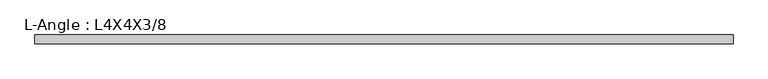
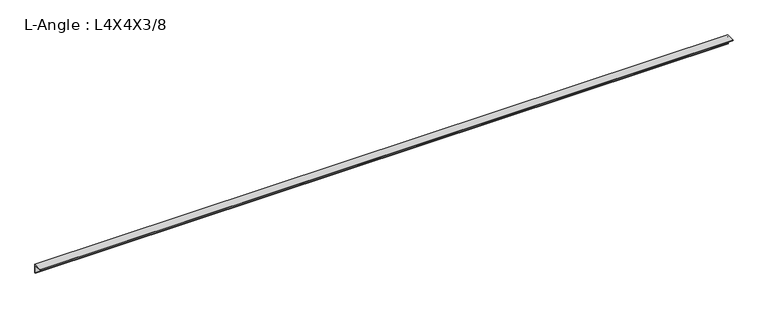
"""IFC4 building model written with IfcOpenShell, lengths in millimetres: beam geometry, L-Angle : L4X4X3/8."""

import ifcopenshell
import ifcopenshell.guid

model = None  # the IFC model being written
_history = None  # IfcOwnerHistory: only IFC2X3 demands one
_inside = {}  # id of a spatial element -> (the spatial element, [elements in it])
_under = {}  # id of a project, library or spatial element -> (it, [spatial elements below it])
_declared = {}  # id of a project -> (the project, [libraries it declares])
_typed = {}  # id of a type object -> (the type object, [elements of that type])
_made_of = {}  # id of a material, layer set ... -> (it, [elements and type objects made of it])


def new_model(schema):
    """Start an empty IFC model of exactly this schema.

    Asked for "IFC4X3", IfcOpenShell would pick the latest addendum, in which some entities
    have other attributes; the version numbers below select the first issue.
    IFC2X3 requires an IfcOwnerHistory on every rooted entity: one is made here for all.
    """
    global model, _history
    if schema == "IFC4X3":
        model = ifcopenshell.file(schema_version=(4, 3, 0, 0))
    else:
        model = ifcopenshell.file(schema=schema)
    _inside.clear()
    _under.clear()
    _declared.clear()
    _typed.clear()
    _made_of.clear()
    _history = None
    if model.schema == "IFC2X3":
        org = make("IfcOrganization", Name="unknown")
        user = make(
            "IfcPersonAndOrganization",
            ThePerson=make("IfcPerson", FamilyName="unknown"),
            TheOrganization=org,
        )
        app = make(
            "IfcApplication",
            ApplicationDeveloper=org,
            Version="unknown",
            ApplicationFullName="unknown",
            ApplicationIdentifier="unknown",
        )
        _history = make(
            "IfcOwnerHistory",
            OwningUser=user,
            OwningApplication=app,
            ChangeAction="ADDED",
            CreationDate=0,
        )
    return model


def make(cls, **values):
    """One entity of the class cls with the attributes given. An attribute that is None is left unset."""
    return model.create_entity(
        cls, **{name: value for name, value in values.items() if value is not None}
    )


def rooted(cls, **values):
    """An entity with a GlobalId (a new one), such as an element, a storey or a relation."""
    return make(cls, GlobalId=ifcopenshell.guid.new(), OwnerHistory=_history, **values)


def si_unit(unit_type, name, prefix=None):
    """IfcSIUnit, for example si_unit("LENGTHUNIT", "METRE", prefix="MILLI")."""
    return make("IfcSIUnit", UnitType=unit_type, Prefix=prefix, Name=name)


def assignment(units):
    """IfcUnitAssignment: the units of a project."""
    return None if units is None else make("IfcUnitAssignment", Units=units)


def point(xyz):
    """IfcCartesianPoint."""
    return None if xyz is None else make("IfcCartesianPoint", Coordinates=xyz)


def direction(xyz):
    """IfcDirection."""
    return None if xyz is None else make("IfcDirection", DirectionRatios=xyz)


def frame(location, z_axis=None, x_axis=None):
    """IfcAxis2Placement3D, a coordinate frame: its origin and axes. An axis left out is left unset."""
    return make(
        "IfcAxis2Placement3D",
        Location=point(location),
        Axis=direction(z_axis),
        RefDirection=direction(x_axis),
    )


def frame_2d(location, x_axis=None):
    """IfcAxis2Placement2D, a coordinate frame in the plane: its origin and x axis."""
    return make(
        "IfcAxis2Placement2D", Location=point(location), RefDirection=direction(x_axis)
    )


def origin():
    """The frame at (0, 0, 0) with its axes left unset."""
    return frame((0.0, 0.0, 0.0))


def place(relative_to, where):
    """IfcLocalPlacement: puts the frame where relative to a parent placement (None: the world)."""
    return make(
        "IfcLocalPlacement", PlacementRelTo=relative_to, RelativePlacement=where
    )


def context(
    kind, dimensions, precision=None, world=None, true_north=None, identifier=None
):
    """IfcGeometricRepresentationContext, for example the 3D "Model" context."""
    return make(
        "IfcGeometricRepresentationContext",
        ContextIdentifier=identifier,
        ContextType=kind,
        CoordinateSpaceDimension=dimensions,
        Precision=precision,
        WorldCoordinateSystem=world,
        TrueNorth=true_north,
    )


def project(units=None, contexts=None):
    """IfcProject with its units and contexts."""
    return rooted(
        "IfcProject",
        Name="project",
        RepresentationContexts=contexts,
        UnitsInContext=assignment(units),
    )


def spatial(cls, under=None, at=None, **own):
    """A site, building, storey or space (cls), placed at a placement, below another one or the project."""
    s = rooted(cls, ObjectPlacement=at, **own)
    if under is not None:
        _under.setdefault(under.id(), (under, []))[1].append(s)
    return s


def polyline(points):
    """IfcPolyline through the points."""
    return make("IfcPolyline", Points=[point(p) for p in points])


def circle_curve(where, radius):
    """IfcCircle in the frame where."""
    return make("IfcCircle", Position=where, Radius=radius)


def trimmed(basis, trim1, trim2, sense, master):
    """IfcTrimmedCurve: the piece of a basis curve between two trims."""
    return make(
        "IfcTrimmedCurve",
        BasisCurve=basis,
        Trim1=trim1,
        Trim2=trim2,
        SenseAgreement=sense,
        MasterRepresentation=master,
    )


def segment(curve, same_sense, transition):
    """IfcCompositeCurveSegment."""
    return make(
        "IfcCompositeCurveSegment",
        Transition=transition,
        SameSense=same_sense,
        ParentCurve=curve,
    )


def composite_curve(segments, self_intersect=None):
    """IfcCompositeCurve: segments joined end to end."""
    return make("IfcCompositeCurve", Segments=segments, SelfIntersect=self_intersect)


def outline(outer, holes=None, kind="AREA"):
    """IfcArbitraryClosedProfileDef: a profile drawn as a closed curve; with holes, ...WithVoids."""
    if holes is None:
        return make("IfcArbitraryClosedProfileDef", ProfileType=kind, OuterCurve=outer)
    return make(
        "IfcArbitraryProfileDefWithVoids",
        ProfileType=kind,
        OuterCurve=outer,
        InnerCurves=holes,
    )


def extrude(swept, where, along, depth):
    """IfcExtrudedAreaSolid: the profile swept, set in the frame where, extruded along a direction by depth."""
    return make(
        "IfcExtrudedAreaSolid",
        SweptArea=swept,
        Position=where,
        ExtrudedDirection=direction(along),
        Depth=depth,
    )


def shape(context_of_items, identifier, shape_type, items):
    """IfcShapeRepresentation: the items that make up one representation, for example the "Body"."""
    return make(
        "IfcShapeRepresentation",
        ContextOfItems=context_of_items,
        RepresentationIdentifier=identifier,
        RepresentationType=shape_type,
        Items=items,
    )


def source(mapping_origin, context_of_items, identifier, shape_type, items):
    """IfcRepresentationMap: a shape defined once, which mapped items show again and again."""
    return make(
        "IfcRepresentationMap",
        MappingOrigin=mapping_origin,
        MappedRepresentation=shape(context_of_items, identifier, shape_type, items),
    )


def transform(
    local_origin,
    x_axis=None,
    y_axis=None,
    z_axis=None,
    scale=None,
    scale2=None,
    scale3=None,
    uniform=True,
):
    """IfcCartesianTransformationOperator3D, or its non-uniform kind. x_axis, y_axis, z_axis: its Axis1, 2, 3."""
    if uniform:
        return make(
            "IfcCartesianTransformationOperator3D",
            Axis1=direction(x_axis),
            Axis2=direction(y_axis),
            LocalOrigin=point(local_origin),
            Scale=scale,
            Axis3=direction(z_axis),
        )
    return make(
        "IfcCartesianTransformationOperator3DnonUniform",
        Axis1=direction(x_axis),
        Axis2=direction(y_axis),
        LocalOrigin=point(local_origin),
        Scale=scale,
        Axis3=direction(z_axis),
        Scale2=scale2,
        Scale3=scale3,
    )


def mapped(mapping_source, mapping_target):
    """IfcMappedItem: shows the shape of a source again, moved by a transform."""
    return make(
        "IfcMappedItem", MappingSource=mapping_source, MappingTarget=mapping_target
    )


def made_of(thing, what):
    """Note that an element or type object is made of a material, layer set ...; save() writes the relation."""
    if what is not None:
        _made_of.setdefault(what.id(), (what, []))[1].append(thing)
    return thing


def element(
    cls,
    number,
    at=None,
    inside=None,
    cuts=None,
    type_object=None,
    material=None,
    context=None,
    identifier="Body",
    shape_type=None,
    held_by="IfcProductDefinitionShape",
    body=None,
    shapes=None,
    **own,
):
    """One element of the class cls, such as IfcWall. Its Tag is "e" and its number.

    at: its placement. inside: the storey or other place that contains it. cuts: it is an
    opening in that element (IfcRelVoidsElement). A single representation is given by context,
    identifier, shape_type and body (its items); several are given by shapes. held_by: the class
    of the entity that holds the representations. save() writes the other relations.
    """
    e = rooted(cls, Tag="e%d" % number, ObjectPlacement=at, **own)
    if body is not None:
        shapes = [shape(context, identifier, shape_type, body)]
    if shapes is not None:
        e.Representation = make(held_by, Representations=shapes)
    if inside is not None:
        _inside.setdefault(inside.id(), (inside, []))[1].append(e)
    if cuts is not None:
        rooted(
            "IfcRelVoidsElement", RelatingBuildingElement=cuts, RelatedOpeningElement=e
        )
    if type_object is not None:
        _typed.setdefault(type_object.id(), (type_object, []))[1].append(e)
    return made_of(e, material)


def aggregate(whole, parts):
    """IfcRelAggregates: a whole, such as a stair, and the parts it consists of."""
    return rooted("IfcRelAggregates", RelatingObject=whole, RelatedObjects=parts)


def save(model, path):
    """Write the relations noted so far, then the file.

    IfcRelAggregates (storeys below a building ...), IfcRelContainedInSpatialStructure (elements
    in a storey), IfcRelDefinesByType, IfcRelAssociatesMaterial and IfcRelDeclares: one each for
    every whole, place, type object, material and project.
    """
    for whole, parts in _under.values():
        aggregate(whole, parts)
    for where, things in _inside.values():
        rooted(
            "IfcRelContainedInSpatialStructure",
            RelatedElements=things,
            RelatingStructure=where,
        )
    for kind, things in _typed.values():
        rooted("IfcRelDefinesByType", RelatedObjects=things, RelatingType=kind)
    for what, things in _made_of.values():
        rooted("IfcRelAssociatesMaterial", RelatedObjects=things, RelatingMaterial=what)
    for by, libraries in _declared.values():
        rooted("IfcRelDeclares", RelatingContext=by, RelatedDefinitions=libraries)
    model.write(path)


def l_angle_l4x4x3_8_194fa828(model_context):
    return source(origin(), model_context, "Body", "SweptSolid", [
        extrude(outline(composite_curve([segment(polyline([(28.702, 28.702), (28.702, -72.898)]), True, "CONTINUOUS"), segment(trimmed(circle_curve(frame_2d((28.702, -63.373)), 9.525), [point((28.702, -72.898))], [point((19.177, -63.373))], False, "CARTESIAN"), True, "CONTINUOUS"), segment(polyline([(19.177, -63.373), (19.177, 9.652)]), True, "CONTINUOUS"), segment(trimmed(circle_curve(frame_2d((9.652, 9.652)), 9.525), [point((19.177, 9.652))], [point((9.652, 19.177))], True, "CARTESIAN"), True, "CONTINUOUS"), segment(polyline([(9.652, 19.177), (-63.373, 19.177)]), True, "CONTINUOUS"), segment(trimmed(circle_curve(frame_2d((-63.373, 28.702)), 9.525), [point((-63.373, 19.177))], [point((-72.898, 28.702))], False, "CARTESIAN"), True, "CONTINUOUS"), segment(polyline([(-72.898, 28.702), (28.702, 28.702)]), True, "CONTINUOUS")], self_intersect=False)), frame((-3919.8223599, 0.0, 0.0), z_axis=(1.0, 0.0, 0.0), x_axis=(0.0, 1.0, 0.0)), (0.0, 0.0, 1.0), 7848.6627754),
    ])


if __name__ == "__main__":
    model = new_model("IFC4")
    model_context = context("Model", 3, world=origin())
    ifc_project = project(units=[si_unit("LENGTHUNIT", "METRE", prefix="MILLI")], contexts=[model_context])
    site = spatial("IfcSite", under=ifc_project)
    building = spatial("IfcBuilding", under=site)
    placement = place(None, origin())
    l_angle_l4x4x3_8_shape = l_angle_l4x4x3_8_194fa828(model_context)
    element("IfcBeam", 1, ObjectType="L-Angle : L4X4X3/8", at=placement, inside=building, context=model_context, shape_type="MappedRepresentation", body=[
        mapped(l_angle_l4x4x3_8_shape, transform((0.0, 0.0, 0.0), x_axis=(1.0, 0.0, 0.0), y_axis=(0.0, 1.0, 0.0), z_axis=(0.0, 0.0, 1.0))),
    ])
    save(model, "model.ifc")

# Revit data of these elements
# Type "L-Angle : L4X4X3/8"
#   Assembly Code = "B10"
#   k = 0' - 0 3/4"
#   W = 9.8
#   Length [instance default] = 5' - 0"
#   b = 0' - 4"
#   d = 0' - 4"
#   t = 0' - 0 3/8"
#   x = 0' - 1.13"
#   y = 0' - 1.13"
#   A = 0.0198611 SF
#   Structural Material [instance default] = Steel ASTM A36
# Element 1 (IfcBeam, "L-Angle : L4X4X3/8")
#   Materials on its faces: "Steel ASTM A36"
# Materials
#   "Steel ASTM A36": class "Metal", colour RGB 199 199 199, transparency 0, Description = "Structural steel, ASTM A36 Grade B, mill finish", Cost = 0
